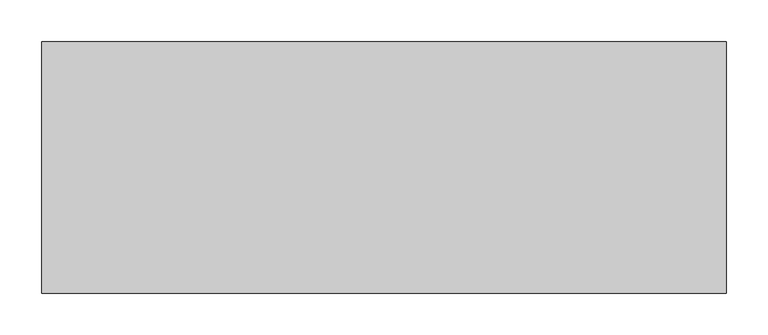
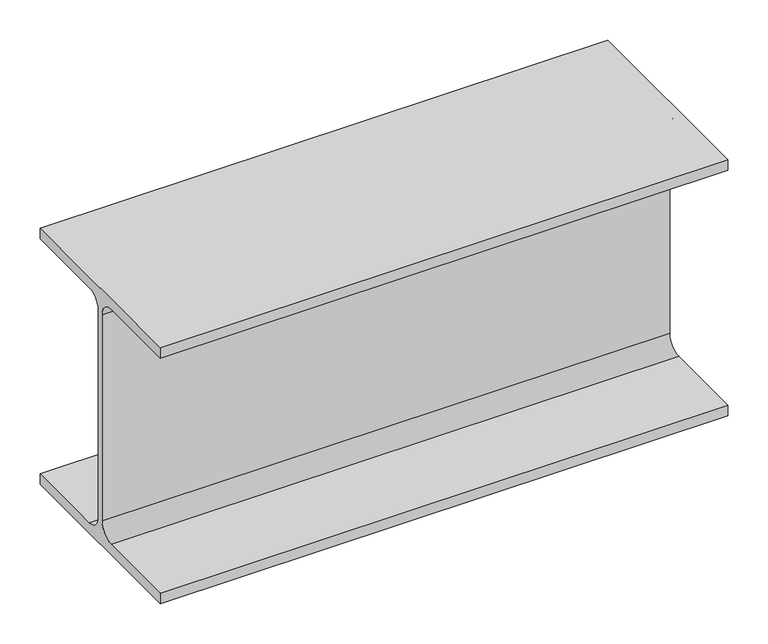
"""IFC4 building model written with IfcOpenShell, lengths in millimetres: beam geometry, 0912_Steel Framing_H-KSD3502 : H_SB_ASB_H-390x300x10x16."""

from ifc_helpers import new_model, si_unit, point, frame, frame_2d, origin, place, context, project, spatial, polyline, circle_curve, trimmed, segment, composite_curve, outline, extrude, source, transform, mapped, element, save


def beam_8d35ebd3(model_context):
    return source(origin(), model_context, "Body", "SweptSolid", [
        extrude(outline(composite_curve([segment(polyline([(150.0, -179.0), (150.0, -195.0), (-150.0, -195.0), (-150.0, -179.0), (-27.0, -179.0)]), True, "CONTINUOUS"), segment(trimmed(circle_curve(frame_2d((-27.0, -157.0)), 22.0), [point((-27.0, -179.0))], [point((-5.0, -157.0))], True, "CARTESIAN"), True, "CONTINUOUS"), segment(polyline([(-5.0, -157.0), (-5.0, 157.0)]), True, "CONTINUOUS"), segment(trimmed(circle_curve(frame_2d((-27.0, 157.0)), 22.0), [point((-5.0, 157.0))], [point((-27.0, 179.0))], True, "CARTESIAN"), True, "CONTINUOUS"), segment(polyline([(-27.0, 179.0), (-150.0, 179.0), (-150.0, 195.0), (150.0, 195.0), (150.0, 179.0), (27.0, 179.0)]), True, "CONTINUOUS"), segment(trimmed(circle_curve(frame_2d((27.0, 157.0)), 22.0), [point((27.0, 179.0))], [point((5.0, 157.0))], True, "CARTESIAN"), True, "CONTINUOUS"), segment(polyline([(5.0, 157.0), (5.0, -157.0)]), True, "CONTINUOUS"), segment(trimmed(circle_curve(frame_2d((27.0, -157.0)), 22.0), [point((5.0, -157.0))], [point((27.0, -179.0))], True, "CARTESIAN"), True, "CONTINUOUS"), segment(polyline([(27.0, -179.0), (150.0, -179.0)]), True, "CONTINUOUS")], self_intersect=False)), frame((-402.2999994, 0.0, 0.0), z_axis=(1.0, 0.0, 0.0), x_axis=(0.0, 1.0, 0.0)), (0.0, 0.0, 1.0), 817.2999994),
    ])


if __name__ == "__main__":
    model = new_model("IFC4")
    model_context = context("Model", 3, world=origin())
    ifc_project = project(units=[si_unit("LENGTHUNIT", "METRE", prefix="MILLI")], contexts=[model_context])
    site = spatial("IfcSite", under=ifc_project)
    building = spatial("IfcBuilding", under=site)
    placement = place(None, origin())
    beam_shape = beam_8d35ebd3(model_context)
    element("IfcBeam", 1, ObjectType="0912_Steel Framing_H-KSD3502 : H_SB_ASB_H-390x300x10x16", at=placement, inside=building, context=model_context, shape_type="MappedRepresentation", body=[
        mapped(beam_shape, transform((0.0, 0.0, 0.0), x_axis=(1.0, 0.0, 0.0), y_axis=(0.0, 1.0, 0.0), z_axis=(0.0, 0.0, 1.0))),
    ])
    save(model, "model.ifc")

# Revit data of these elements
# Type "0912_Steel Framing_H-KSD3502 : H_SB_ASB_H-390x300x10x16"
#   H_WM Code_1 = "S01AA001-00001 | Main Steel Structure Fabrication Work | Shelter/Building | Heavy Steel - Standard (Weight≥90KG/M) | Material: (   )"
#   H_WM Code_2 = "S03AA027-00001 | Main Steel Structure Erection Work | Shelter/Building | Heavy Steel (Weight≥90KG/M) | Material: (   )"
#   H_WM Code_3 = "S01AA010-00001 | Main Steel Structure Fabrication Work | Shelter/Building | Steel Painting/Coating | for Non-Fireproofed Steel Surface, Surface Preparation, Primer, Second & Final Coat | Material: (   )"
#   H_Q'ty Cal Type Tag = "SB-Q2"
#   Width = 30.0 cm
#   Web Thickness = 1.0 cm
#   Web Fillet = 2.2 cm
#   Warping Constant = 2520000.0 cm⁶
#   W = 0
#   Torsional Moment of Inertia = 94.3867 cm⁴
#   Section Area = 136.0 cm²
#   Plastic Modulus weak axis = 733.0 cm³
#   Plastic Modulus strong axis = 2190.0 cm³
#   Perimeter = 1.92 m²/m
#   Nominal Weight = 107.00 kgf/m
#   Moment of Inertia weak axis = 7210.00 cm⁴
#   Moment of Inertia strong axis = 38700.00 cm⁴
#   Height = 39.0 cm
#   Flange Thickness = 1.6 cm
#   Elastic Modulus weak axis = 481.0 cm³
#   Elastic Modulus strong axis = 1980.0 cm³
#   Centroid Vertical = 19.5 cm
#   Centroid Horizontal = 15.0 cm
#   Ix = 387000000
#   Length [instance default] = 1.5240 m
#   Zx = 2190000
#   b = 0.3000 m
#   h = 0.3900 m
#   r = 0.0220 m
#   s = 0.0100 m
#   t = 0.0160 m
#   A = 0.0136 m²
#   Structural Material [instance default] = Steel, 45-345
#   Assembly Code = ""
# Element 1 (IfcBeam, "0912_Steel Framing_H-KSD3502 : H_SB_ASB_H-390x300x10x16")
#   Structural Material = none
# Materials
#   "Steel, 45-345": class "Metal", colour RGB 189 187 185, transparency 0, Description = "Steel 345 MPa", Cost = 0
